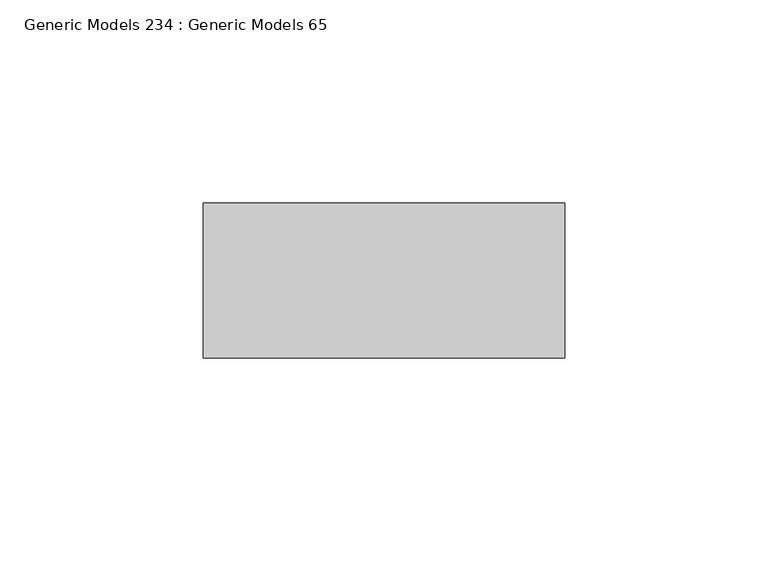
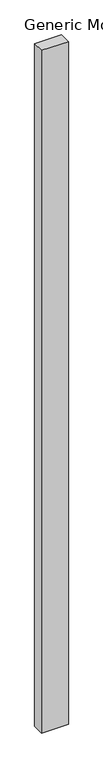
"""IFC4 building model written with IfcOpenShell, lengths in millimetres: proxy geometry, Generic Models 234 : Generic Models 65."""

from ifc_helpers import new_model, si_unit, frame, origin, place, context, project, spatial, polyline, outline, extrude, source, transform, mapped, element, save


def generic_models_234_generic_models_65_886ed74c(model_context):
    return source(origin(), model_context, "Body", "SweptSolid", [
        extrude(outline(polyline([(49784.0, 592.1375), (49695.1, 592.1375), (49695.1, 630.2375), (49784.0, 630.2375), (49784.0, 592.1375)])), frame((0.0, 0.0, 3086.1), z_axis=(0.0, 0.0, 1.0), x_axis=(1.0, 0.0, 0.0)), (0.0, 0.0, 1.0), 2381.25),
    ])


if __name__ == "__main__":
    model = new_model("IFC4")
    model_context = context("Model", 3, world=origin())
    ifc_project = project(units=[si_unit("LENGTHUNIT", "METRE", prefix="MILLI")], contexts=[model_context])
    site = spatial("IfcSite", under=ifc_project)
    building = spatial("IfcBuilding", under=site)
    placement = place(None, origin())
    generic_models_234_generic_models_65_shape = generic_models_234_generic_models_65_886ed74c(model_context)
    element("IfcBuildingElementProxy", 1, Name="Generic Models 234 : Generic Models 65", ObjectType="Generic Models 234 : Generic Models 65", at=placement, inside=building, context=model_context, shape_type="MappedRepresentation", body=[
        mapped(generic_models_234_generic_models_65_shape, transform((0.0, 0.0, 0.0), x_axis=(1.0, 0.0, 0.0), y_axis=(0.0, 1.0, 0.0), z_axis=(0.0, 0.0, 1.0))),
    ])
    save(model, "model.ifc")

# Revit data of these elements
# Element 1 (IfcBuildingElementProxy, "Generic Models 234 : Generic Models 65")
#   Materials on its faces: "2X WOOD STUD - SEE 'WALL TAG' & 'LAYER MATERIAL SCHEDULE' FOR SPACING & INSULATION TREATMENT, IF APPLICAPLE"
# Materials
#   "2X WOOD STUD - SEE 'WALL TAG' & 'LAYER MATERIAL SCHEDULE' FOR SPACING & INSULATION TREATMENT, IF APPLICAPLE": class "Wood", colour RGB 234 198 147, transparency 0, Description = "Pinus Echinata", Cost = 0
